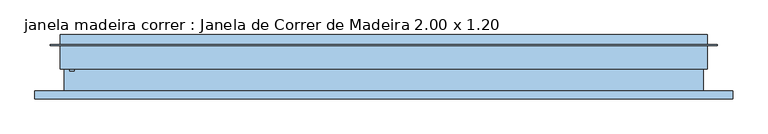
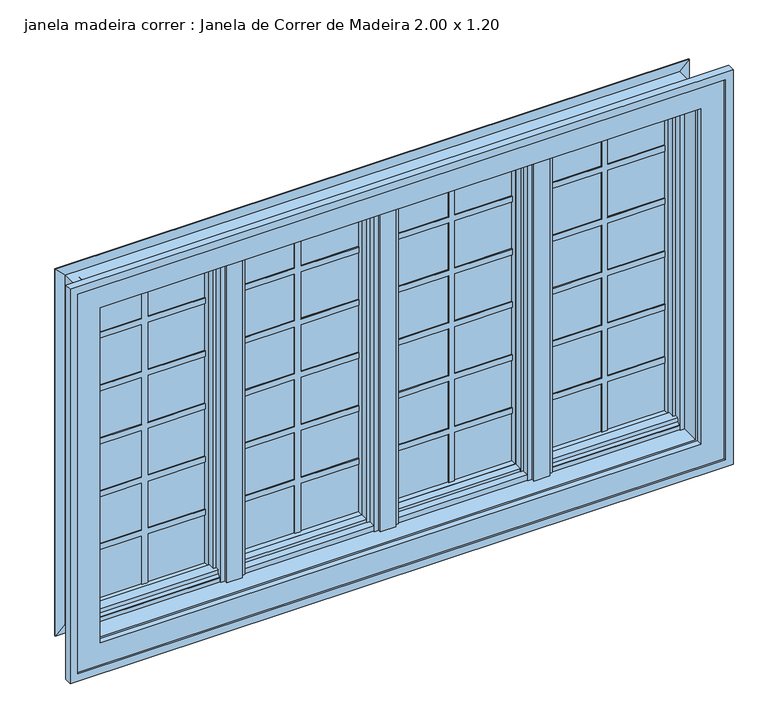
"""IFC4 building model written with IfcOpenShell, lengths in millimetres: window geometry, janela madeira correr : Janela de Correr de Madeira 2.00 x 1.20."""

from ifc_helpers import new_model, si_unit, frame, origin, place, context, project, spatial, polyline, outline, extrude, faceted_brep, source, transform, mapped, element, save


def janela_madeira_correr_janela_de_correr_de_madeira_2_00_x_1_d447c460(model_context):
    return source(origin(), model_context, "Body", "SolidModel", [
        extrude(outline(polyline([(1881.6300584, 206.5264803), (1881.6300584, 13.2337398), (1862.5800584, 13.2337398), (1862.5800584, 206.5264803), (1699.6775292, 206.5264803), (1699.6775292, 13.2337398), (1680.6275292, 13.2337398), (1680.6275292, 206.5264803), (1517.725, 206.5264803), (1517.725, 13.2337398), (1498.675, 13.2337398), (1498.675, 206.5264803), (1335.7724708, 206.5264803), (1335.7724708, 13.2337398), (1316.7224708, 13.2337398), (1316.7224708, 206.5264803), (1153.8199416, 206.5264803), (1153.8199416, 13.2337398), (1134.7699416, 13.2337398), (1134.7699416, 206.5264803), (962.3424123, 206.5264803), (962.3424123, 225.5764803), (1134.7699416, 225.5764803), (1134.7699416, 418.8692207), (1153.8199416, 418.8692207), (1153.8199416, 225.5764803), (1316.7224708, 225.5764803), (1316.7224708, 418.8692207), (1335.7724708, 418.8692207), (1335.7724708, 225.5764803), (1498.675, 225.5764803), (1498.675, 418.8692207), (1517.725, 418.8692207), (1517.725, 225.5764803), (1680.6275292, 225.5764803), (1680.6275292, 418.8692207), (1699.6775292, 418.8692207), (1699.6775292, 225.5764803), (1862.5800584, 225.5764803), (1862.5800584, 418.8692207), (1881.6300584, 418.8692207), (1881.6300584, 225.5764803), (2054.0575877, 225.5764803), (2054.0575877, 206.5264803), (1881.6300584, 206.5264803)])), frame((0.0, 46.9582456, 0.0), z_axis=(0.0, 1.0, 0.0), x_axis=(0.0, 0.0, 1.0)), (0.0, 0.0, 1.0), 3.1432544),
        extrude(outline(polyline([(1881.6300584, -293.4735197), (1881.6300584, -486.7662602), (1862.5800584, -486.7662602), (1862.5800584, -293.4735197), (1699.6775292, -293.4735197), (1699.6775292, -486.7662602), (1680.6275292, -486.7662602), (1680.6275292, -293.4735197), (1517.725, -293.4735197), (1517.725, -486.7662602), (1498.675, -486.7662602), (1498.675, -293.4735197), (1335.7724708, -293.4735197), (1335.7724708, -486.7662602), (1316.7224708, -486.7662602), (1316.7224708, -293.4735197), (1153.8199416, -293.4735197), (1153.8199416, -486.7662602), (1134.7699416, -486.7662602), (1134.7699416, -293.4735197), (962.3424123, -293.4735197), (962.3424123, -274.4235197), (1134.7699416, -274.4235197), (1134.7699416, -81.1307793), (1153.8199416, -81.1307793), (1153.8199416, -274.4235197), (1316.7224708, -274.4235197), (1316.7224708, -81.1307793), (1335.7724708, -81.1307793), (1335.7724708, -274.4235197), (1498.675, -274.4235197), (1498.675, -81.1307793), (1517.725, -81.1307793), (1517.725, -274.4235197), (1680.6275292, -274.4235197), (1680.6275292, -81.1307793), (1699.6775292, -81.1307793), (1699.6775292, -274.4235197), (1862.5800584, -274.4235197), (1862.5800584, -81.1307793), (1881.6300584, -81.1307793), (1881.6300584, -274.4235197), (2054.0575877, -274.4235197), (2054.0575877, -293.4735197), (1881.6300584, -293.4735197)])), frame((0.0, 46.9582456, 0.0), z_axis=(0.0, 1.0, 0.0), x_axis=(0.0, 0.0, 1.0)), (0.0, 0.0, 1.0), 3.1432544),
        extrude(outline(polyline([(1881.6300584, 206.5264803), (1881.6300584, 13.2337398), (1862.5800584, 13.2337398), (1862.5800584, 206.5264803), (1699.6775292, 206.5264803), (1699.6775292, 13.2337398), (1680.6275292, 13.2337398), (1680.6275292, 206.5264803), (1517.725, 206.5264803), (1517.725, 13.2337398), (1498.675, 13.2337398), (1498.675, 206.5264803), (1335.7724708, 206.5264803), (1335.7724708, 13.2337398), (1316.7224708, 13.2337398), (1316.7224708, 206.5264803), (1153.6503822, 206.5264803), (1153.6503822, 13.2337398), (1134.6003822, 13.2337398), (1134.6003822, 206.5264803), (962.3424123, 206.5264803), (962.3424123, 225.5764803), (1134.6003822, 225.5764803), (1134.6003822, 418.8692207), (1153.6503822, 418.8692207), (1153.6503822, 225.5764803), (1316.7224708, 225.5764803), (1316.7224708, 418.8692207), (1335.7724708, 418.8692207), (1335.7724708, 225.5764803), (1498.675, 225.5764803), (1498.675, 418.8692207), (1517.725, 418.8692207), (1517.725, 225.5764803), (1680.6275292, 225.5764803), (1680.6275292, 418.8692207), (1699.6775292, 418.8692207), (1699.6775292, 225.5764803), (1862.5800584, 225.5764803), (1862.5800584, 418.8692207), (1881.6300584, 418.8692207), (1881.6300584, 225.5764803), (2054.0575877, 225.5764803), (2054.0575877, 206.5264803), (1881.6300584, 206.5264803)])), frame((0.0, 50.1015, 0.0), z_axis=(0.0, 1.0, 0.0), x_axis=(0.0, 0.0, 1.0)), (0.0, 0.0, 1.0), 15.875),
        extrude(outline(polyline([(1881.6300584, -293.4735197), (1881.6300584, -486.7662602), (1862.5800584, -486.7662602), (1862.5800584, -293.4735197), (1699.6775292, -293.4735197), (1699.6775292, -486.7662602), (1680.6275292, -486.7662602), (1680.6275292, -293.4735197), (1517.725, -293.4735197), (1517.725, -486.7662602), (1498.675, -486.7662602), (1498.675, -293.4735197), (1335.7724708, -293.4735197), (1335.7724708, -486.7662602), (1316.7224708, -486.7662602), (1316.7224708, -293.4735197), (1153.8199416, -293.4735197), (1153.8199416, -486.7662602), (1134.7699416, -486.7662602), (1134.7699416, -293.4735197), (962.3424123, -293.4735197), (962.3424123, -274.4235197), (1134.7699416, -274.4235197), (1134.7699416, -81.1307793), (1153.8199416, -81.1307793), (1153.8199416, -274.4235197), (1316.7224708, -274.4235197), (1316.7224708, -81.1307793), (1335.7724708, -81.1307793), (1335.7724708, -274.4235197), (1498.675, -274.4235197), (1498.675, -81.1307793), (1517.725, -81.1307793), (1517.725, -274.4235197), (1680.6275292, -274.4235197), (1680.6275292, -81.1307793), (1699.6775292, -81.1307793), (1699.6775292, -274.4235197), (1862.5800584, -274.4235197), (1862.5800584, -81.1307793), (1881.6300584, -81.1307793), (1881.6300584, -274.4235197), (2054.0575877, -274.4235197), (2054.0575877, -293.4735197), (1881.6300584, -293.4735197)])), frame((0.0, 50.1015, 0.0), z_axis=(0.0, 1.0, 0.0), x_axis=(0.0, 0.0, 1.0)), (0.0, 0.0, 1.0), 15.875),
        extrude(outline(polyline([(-79.1922697, 50.1015), (-488.7047697, 50.1015), (-488.7047697, 65.9765), (-79.1922697, 65.9765), (-79.1922697, 50.1015)])), frame((0.0, 0.0, 962.3424123), z_axis=(0.0, 0.0, 1.0), x_axis=(1.0, 0.0, 0.0)), (0.0, 0.0, 1.0), 1091.7151753),
        faceted_brep([(1019.5438803, -105.0, 855.00605), (1019.5438803, -98.65, 855.00605), (-1087.4409197, -98.65, 855.00605), (-1087.4409197, -105.0, 855.00605), (1044.9438803, -79.6, 829.60605), (1044.9438803, -105.0, 829.60605), (-1112.8409197, -105.0, 829.60605), (-1112.8409197, -79.6, 829.60605), (943.3438803, -98.65, 931.20605), (943.3438803, -79.6, 931.20605), (-1011.2409197, -79.6, 931.20605), (-1011.2409197, -98.65, 931.20605), (-1087.4409197, -98.65, 2161.72415), (-1087.4409197, -105.0, 2161.72415), (-1112.8409197, -105.0, 2187.12415), (-1112.8409197, -79.6, 2187.12415), (-1011.2409197, -79.6, 2085.52415), (-1011.2409197, -98.65, 2085.52415), (1019.5438803, -98.65, 2161.72415), (1019.5438803, -105.0, 2161.72415), (1044.9438803, -105.0, 2187.12415), (1044.9438803, -79.6, 2187.12415), (943.3438803, -79.6, 2085.52415), (943.3438803, -98.65, 2085.52415)], [[[0, 1, 2, 3]], [[4, 5, 6, 7]], [[8, 9, 10, 11]], [[3, 2, 12, 13]], [[7, 6, 14, 15]], [[11, 10, 16, 17]], [[13, 12, 18, 19]], [[15, 14, 20, 21]], [[17, 16, 22, 23]], [[1, 18, 12, 2], [11, 17, 23, 8]], [[19, 18, 1, 0]], [[5, 20, 14, 6], [3, 13, 19, 0]], [[21, 20, 5, 4]], [[7, 15, 21, 4], [9, 22, 16, 10]], [[23, 22, 9, 8]]]),
        extrude(outline(polyline([(1153.8199416, 723.716552), (1316.7224708, 723.716552), (1316.7224708, 917.0878737), (1335.7724708, 917.0878737), (1335.7724708, 723.716552), (1498.675, 723.716552), (1498.675, 917.0878737), (1517.725, 917.0878737), (1517.725, 723.716552), (1680.6275292, 723.716552), (1680.6275292, 917.0878737), (1699.6775292, 917.0878737), (1699.6775292, 723.716552), (1862.5800584, 723.716552), (1862.5800584, 917.0878737), (1881.6300584, 917.0878737), (1881.6300584, 723.716552), (2054.0575877, 723.716552), (2054.0575877, 704.666552), (1881.6300584, 704.666552), (1881.6300584, 511.2952303), (1862.5800584, 511.2952303), (1862.5800584, 704.666552), (1699.6775292, 704.666552), (1699.6775292, 511.2952303), (1680.6275292, 511.2952303), (1680.6275292, 704.666552), (1517.725, 704.666552), (1517.725, 511.2952303), (1498.675, 511.2952303), (1498.675, 704.666552), (1335.7724708, 704.666552), (1335.7724708, 511.2952303), (1316.7224708, 511.2952303), (1316.7224708, 704.666552), (1153.8199416, 704.666552), (1153.8199416, 511.2952303), (1134.7699416, 511.2952303), (1134.7699416, 704.666552), (962.3424123, 704.666552), (962.3424123, 723.716552), (1134.7699416, 723.716552), (1134.7699416, 917.0878737), (1153.8199416, 917.0878737), (1153.8199416, 723.716552)])), frame((0.0, 46.7303732, 0.0), z_axis=(0.0, 1.0, 0.0), x_axis=(0.0, 0.0, 1.0)), (0.0, 0.0, 1.0), 3.3711268),
        extrude(outline(polyline([(1881.6300584, -791.6417168), (1881.6300584, -984.9344572), (1862.5800584, -984.9344572), (1862.5800584, -791.6417168), (1699.6775292, -791.6417168), (1699.6775292, -984.9344572), (1680.6275292, -984.9344572), (1680.6275292, -791.6417168), (1517.725, -791.6417168), (1517.725, -984.9344572), (1498.675, -984.9344572), (1498.675, -791.6417168), (1335.7724708, -791.6417168), (1335.7724708, -984.9344572), (1316.7224708, -984.9344572), (1316.7224708, -791.6417168), (1153.8199416, -791.6417168), (1153.8199416, -984.9344572), (1134.7699416, -984.9344572), (1134.7699416, -791.6417168), (962.3424123, -791.6417168), (962.3424123, -772.5917168), (1134.7699416, -772.5917168), (1134.7699416, -579.2989763), (1153.8199416, -579.2989763), (1153.8199416, -772.5917168), (1316.7224708, -772.5917168), (1316.7224708, -579.2989763), (1335.7724708, -579.2989763), (1335.7724708, -772.5917168), (1498.675, -772.5917168), (1498.675, -579.2989763), (1517.725, -579.2989763), (1517.725, -772.5917168), (1680.6275292, -772.5917168), (1680.6275292, -579.2989763), (1699.6775292, -579.2989763), (1699.6775292, -772.5917168), (1862.5800584, -772.5917168), (1862.5800584, -579.2989763), (1881.6300584, -579.2989763), (1881.6300584, -772.5917168), (2054.0575877, -772.5917168), (2054.0575877, -791.6417168), (1881.6300584, -791.6417168)])), frame((0.0, 46.9582456, 0.0), z_axis=(0.0, 1.0, 0.0), x_axis=(0.0, 0.0, 1.0)), (0.0, 0.0, 1.0), 3.1432544),
        extrude(outline(polyline([(35.1373, 2049.7546), (9.8065079, 2049.7546), (9.2928, 2058.8986), (-15.6627, 2058.8986), (-15.6627, 2079.17415), (-11.7892, 2079.17415), (-11.7892, 2072.0304), (35.1373, 2072.0304), (35.1373, 2049.7546)])), frame((-494.6547197, 0.0, 0.0), z_axis=(1.0, 0.0, 0.0), x_axis=(0.0, 1.0, 0.0)), (0.0, 0.0, 1.0), 921.4124),
        extrude(outline(polyline([(35.1373, 965.477), (35.1373, 944.3696), (-11.7892, 944.3696), (-11.7892, 937.55605), (-15.6627, 937.55605), (-15.6627, 955.952), (9.0471115, 955.952), (9.8065079, 965.477), (35.1373, 965.477)])), frame((-494.6547197, 0.0, 0.0), z_axis=(1.0, 0.0, 0.0), x_axis=(0.0, 1.0, 0.0)), (0.0, 0.0, 1.0), 921.4124),
        extrude(outline(polyline([(35.1373, 2049.7546), (9.8065079, 2049.7546), (9.2928, 2058.8986), (-15.6627, 2058.8986), (-15.6627, 2079.17415), (-11.7892, 2079.17415), (-11.7892, 2072.0304), (35.1373, 2072.0304), (35.1373, 2049.7546)])), frame((-990.9971197, 0.0, 0.0), z_axis=(1.0, 0.0, 0.0), x_axis=(0.0, 1.0, 0.0)), (0.0, 0.0, 1.0), 417.6462326),
        extrude(outline(polyline([(35.1373, 965.477), (35.1373, 944.3696), (-11.7892, 944.3696), (-11.7892, 937.55605), (-15.6627, 937.55605), (-15.6627, 951.5578), (-12.2972, 951.5578), (-5.0582, 959.4826), (-3.9768196, 973.0462), (27.9364, 973.0462), (35.1373, 965.477)])), frame((-990.9971197, 0.0, 0.0), z_axis=(1.0, 0.0, 0.0), x_axis=(0.0, 1.0, 0.0)), (0.0, 0.0, 1.0), 417.6462326),
        faceted_brep([(454.9389803, 85.9373, 2088.2955442), (454.9389803, 48.6374, 2088.2955442), (454.9389803, 48.6374, 2069.8909496), (454.9389803, 35.1373, 2067.5291599), (454.9389803, 35.1373, 2050.1057516), (454.9389803, 48.6374, 2047.8865571), (454.9389803, 48.6374, 968.5290777), (454.9389803, 35.1373, 966.3098832), (454.9389803, 35.1373, 948.8864749), (454.9389803, 48.6374, 946.5246852), (454.9389803, 48.6374, 928.1044558), (454.9389803, 85.9373, 928.1044558), (-23.7161471, 85.9373, 2088.2955442), (-23.7161471, 85.9373, 2059.2701124), (-23.7161471, 74.7560374, 2057.8452835), (-23.7161471, 74.4029109, 2047.2338554), (-23.7161471, 69.3765, 2044.5482224), (-23.7161471, 69.3765, 2060.523579), (-23.7161471, 53.5015, 2060.523579), (-23.7161471, 53.5015, 2047.086979), (-23.7161471, 35.1373, 2050.1057516), (-23.7161471, 35.1373, 2067.5291599), (-23.7161471, 48.6374, 2069.8909496), (-23.7161471, 48.6374, 2088.2955442), (-23.7161471, 53.5015, 969.3286558), (-23.7161471, 53.5015, 955.8920558), (-23.7161471, 69.3765, 955.8920558), (-23.7161471, 69.3765, 971.8674123), (-23.7161471, 74.4029109, 969.1817794), (-23.7161471, 74.7560374, 958.5703513), (-23.7161471, 85.9373, 957.1455224), (-23.7161471, 85.9373, 928.1044558), (-23.7161471, 48.6374, 928.1044558), (-23.7161471, 48.6374, 946.5246852), (-23.7161471, 35.1373, 948.8864749), (-23.7161471, 35.1373, 966.3098832), (-4.4157903, 48.6374, 2088.2955442), (-2.0540006, 35.1373, 2088.2955442), (15.3694077, 35.1373, 2088.2955442), (17.5886022, 48.6374, 2088.2955442), (414.5143584, 48.6374, 2088.2955442), (416.7335529, 35.1373, 2088.2955442), (434.1569612, 35.1373, 2088.2955442), (436.5187509, 48.6374, 2088.2955442), (436.5187509, 48.6374, 2069.8909496), (-22.8360197, 48.6374, 2069.8909496), (-4.4157903, 48.6374, 2069.8909496), (17.5886022, 48.6374, 2069.8909496), (414.5143584, 48.6374, 2069.8909496), (434.1569612, 35.1373, 2067.5291599), (-2.0540006, 35.1373, 2067.5291599), (15.3694077, 35.1373, 2067.5291599), (416.7335529, 35.1373, 2067.5291599), (-2.0540006, 35.1373, 928.1044558), (15.3694077, 35.1373, 928.1044558), (15.3694077, 35.1373, 948.8864749), (416.7335529, 35.1373, 948.8864749), (416.7335529, 35.1373, 928.1044558), (434.1569612, 35.1373, 928.1044558), (434.1569612, 35.1373, 948.8864749), (434.1569612, 35.1373, 966.3098832), (434.1569612, 35.1373, 2050.1057516), (-2.0540006, 35.1373, 2050.1057516), (-2.0540006, 35.1373, 966.3098832), (-2.0540006, 35.1373, 948.8864749), (416.7335529, 35.1373, 2050.1057516), (416.7335529, 35.1373, 966.3098832), (15.3694077, 35.1373, 966.3098832), (15.3694077, 35.1373, 2050.1057516), (436.5187509, 48.6374, 2047.8865571), (-22.8360197, 53.5015, 2047.086979), (-22.8360197, 48.6374, 2047.8865571), (-4.4157903, 48.6374, 2047.8865571), (18.3881803, 53.5015, 2047.086979), (413.7147803, 53.5015, 2047.086979), (-22.8360197, 53.5015, 2060.523579), (-22.8360197, 53.5015, 969.3286558), (-22.8360197, 53.5015, 955.8920558), (427.1513803, 53.5015, 2060.523579), (427.1513803, 53.5015, 955.8920558), (4.9515803, 53.5015, 955.8920558), (4.9515803, 53.5015, 2060.523579), (18.3881803, 53.5015, 969.3286558), (413.7147803, 53.5015, 969.3286558), (-22.8360197, 69.3765, 2060.523579), (4.9515803, 69.3765, 2060.523579), (427.1513803, 69.3765, 2060.523579), (-22.8360197, 69.3765, 2044.5482224), (-22.8360197, 69.3765, 955.8920558), (-22.8360197, 69.3765, 971.8674123), (4.9515803, 69.3765, 955.8920558), (427.1513803, 69.3765, 955.8920558), (411.1760237, 69.3765, 2044.5482224), (411.1760237, 69.3765, 971.8674123), (20.9269368, 69.3765, 971.8674123), (20.9269368, 69.3765, 2044.5482224), (-22.8360197, 74.4029109, 2047.2338554), (18.2413039, 74.4029109, 2047.2338554), (413.8616566, 74.4029109, 2047.2338554), (-22.8360197, 74.7560374, 2057.8452835), (7.6298758, 74.7560374, 2057.8452835), (424.4730847, 74.7560374, 2057.8452835), (-22.8360197, 85.9373, 2059.2701124), (6.2050469, 85.9373, 2059.2701124), (425.8979136, 85.9373, 2059.2701124), (-22.8360197, 85.9373, 957.1455224), (6.2050469, 85.9373, 957.1455224), (425.8979136, 85.9373, 957.1455224), (436.5187509, 48.6374, 968.5290777), (-4.4157903, 48.6374, 968.5290777), (-22.8360197, 48.6374, 968.5290777), (436.5187509, 48.6374, 946.5246852), (-22.8360197, 48.6374, 946.5246852), (-4.4157903, 48.6374, 946.5246852), (17.5886022, 48.6374, 946.5246852), (414.5143584, 48.6374, 946.5246852), (436.5187509, 48.6374, 928.1044558), (-4.4157903, 48.6374, 928.1044558), (17.5886022, 48.6374, 928.1044558), (414.5143584, 48.6374, 928.1044558), (-22.8360197, 74.7560374, 958.5703513), (7.6298758, 74.7560374, 958.5703513), (424.4730847, 74.7560374, 958.5703513), (-22.8360197, 74.4029109, 969.1817794), (18.2413039, 74.4029109, 969.1817794), (413.8616566, 74.4029109, 969.1817794)], [[[0, 1, 2, 3, 4, 5, 6, 7, 8, 9, 10, 11]], [[12, 13, 14, 15, 16, 17, 18, 19, 20, 21, 22, 23]], [[24, 25, 26, 27, 28, 29, 30, 31, 32, 33, 34, 35]], [[1, 0, 12, 23, 36, 37, 38, 39, 40, 41, 42, 43]], [[2, 1, 43, 44]], [[36, 23, 22, 45, 46]], [[40, 39, 47, 48]], [[3, 2, 44, 49]], [[22, 21, 50, 46, 45]], [[48, 47, 51, 52]], [[53, 54, 55, 56, 57, 58, 59, 8, 7, 60, 61, 4, 3, 49, 42, 41, 52, 51, 38, 37, 50, 21, 20, 62, 63, 35, 34, 64], [65, 66, 67, 68]], [[5, 4, 61, 69]], [[20, 19, 70, 71, 72, 62]], [[65, 68, 73, 74]], [[19, 18, 75, 70]], [[25, 24, 76, 77]], [[78, 79, 80, 81], [74, 73, 82, 83]], [[18, 17, 84, 75]], [[78, 81, 85, 86]], [[17, 16, 87, 84]], [[27, 26, 88, 89]], [[86, 85, 90, 91], [92, 93, 94, 95]], [[16, 15, 96, 87]], [[92, 95, 97, 98]], [[15, 14, 99, 96]], [[98, 97, 100, 101]], [[14, 13, 102, 99]], [[101, 100, 103, 104]], [[12, 0, 11, 31, 30, 105, 102, 13], [103, 106, 107, 104]], [[7, 6, 108, 60]], [[24, 35, 63, 109, 110, 76]], [[83, 82, 67, 66]], [[9, 8, 59, 111]], [[34, 33, 112, 113, 64]], [[56, 55, 114, 115]], [[10, 9, 111, 116]], [[33, 32, 117, 113, 112]], [[115, 114, 118, 119]], [[31, 11, 10, 116, 58, 57, 119, 118, 54, 53, 117, 32]], [[30, 29, 120, 105]], [[107, 106, 121, 122]], [[29, 28, 123, 120]], [[122, 121, 124, 125]], [[28, 27, 89, 123]], [[125, 124, 94, 93]], [[26, 25, 77, 88]], [[91, 90, 80, 79]], [[101, 122, 125, 98]], [[104, 107, 122, 101]], [[6, 5, 69, 108]], [[43, 42, 49, 44]], [[61, 60, 108, 69]], [[58, 116, 111, 59]], [[41, 40, 48, 52]], [[57, 56, 115, 119]], [[74, 83, 66, 65]], [[79, 78, 86, 91]], [[98, 125, 93, 92]], [[124, 97, 95, 94]], [[81, 80, 90, 85]], [[39, 38, 51, 47]], [[55, 54, 118, 114]], [[82, 73, 68, 67]], [[37, 36, 46, 50]], [[63, 62, 72, 109]], [[117, 53, 64, 113]], [[109, 72, 71, 110]], [[102, 105, 120, 123, 89, 88, 77, 76, 110, 71, 70, 75, 84, 87, 96, 99]], [[106, 103, 100, 121]], [[121, 100, 97, 124]]]),
        faceted_brep([(-86.1383434, 74.4029109, 2088.2955442), (-88.8239763, 69.3765, 2088.2955442), (-72.8486197, 69.3765, 2088.2955442), (-72.8486197, 53.5015, 2088.2955442), (-86.2852197, 53.5015, 2088.2955442), (-83.2664471, 35.1373, 2088.2955442), (-65.8430388, 35.1373, 2088.2955442), (-63.4812491, 48.6374, 2088.2955442), (-45.0610197, 48.6374, 2088.2955442), (-45.0610197, 85.9373, 2088.2955442), (-74.1020864, 85.9373, 2088.2955442), (-75.5269153, 74.7560374, 2088.2955442), (-86.1383434, 74.4029109, 928.1044558), (-75.5269153, 74.7560374, 928.1044558), (-74.1020864, 85.9373, 928.1044558), (-45.0610197, 85.9373, 928.1044558), (-45.0610197, 48.6374, 928.1044558), (-63.4812491, 48.6374, 928.1044558), (-65.8430388, 35.1373, 928.1044558), (-83.2664471, 35.1373, 928.1044558), (-86.2852197, 53.5015, 928.1044558), (-72.8486197, 53.5015, 928.1044558), (-72.8486197, 69.3765, 928.1044558), (-88.8239763, 69.3765, 928.1044558)], [[[0, 1, 2, 3, 4, 5, 6, 7, 8, 9, 10, 11]], [[12, 13, 14, 15, 16, 17, 18, 19, 20, 21, 22, 23]], [[13, 12, 0, 11]], [[14, 13, 11, 10]], [[15, 14, 10, 9]], [[16, 15, 9, 8]], [[17, 16, 8, 7]], [[18, 17, 7, 6]], [[19, 18, 6, 5]], [[20, 19, 5, 4]], [[21, 20, 4, 3]], [[22, 21, 3, 2]], [[23, 22, 2, 1]], [[12, 23, 1, 0]]]),
        faceted_brep([(-481.7586961, 74.4029109, 2088.2955442), (-492.3701242, 74.7560374, 2088.2955442), (-493.7949531, 85.9373, 2088.2955442), (-522.8360197, 85.9373, 2088.2955442), (-522.8360197, 48.6374, 2088.2955442), (-504.4157903, 48.6374, 2088.2955442), (-502.0540006, 35.1373, 2088.2955442), (-484.6305923, 35.1373, 2088.2955442), (-481.6118197, 53.5015, 2088.2955442), (-495.0484197, 53.5015, 2088.2955442), (-495.0484197, 69.3765, 2088.2955442), (-479.0730632, 69.3765, 2088.2955442), (-481.7586961, 74.4029109, 928.1044558), (-479.0730632, 69.3765, 928.1044558), (-495.0484197, 69.3765, 928.1044558), (-495.0484197, 53.5015, 928.1044558), (-481.6118197, 53.5015, 928.1044558), (-484.6305923, 35.1373, 928.1044558), (-502.0540006, 35.1373, 928.1044558), (-504.4157903, 48.6374, 928.1044558), (-522.8360197, 48.6374, 928.1044558), (-522.8360197, 85.9373, 928.1044558), (-493.7949531, 85.9373, 928.1044558), (-492.3701242, 74.7560374, 928.1044558)], [[[0, 1, 2, 3, 4, 5, 6, 7, 8, 9, 10, 11]], [[12, 13, 14, 15, 16, 17, 18, 19, 20, 21, 22, 23]], [[13, 12, 0, 11]], [[14, 13, 11, 10]], [[15, 14, 10, 9]], [[16, 15, 9, 8]], [[17, 16, 8, 7]], [[18, 17, 7, 6]], [[19, 18, 6, 5]], [[20, 19, 5, 4]], [[21, 20, 4, 3]], [[22, 21, 3, 2]], [[23, 22, 2, 1]], [[12, 23, 1, 0]]]),
        extrude(outline(polyline([(35.1373, 2049.7546), (9.8065079, 2049.7546), (9.2928, 2058.8986), (-15.6627, 2058.8986), (-15.6627, 2079.17415), (-11.7892, 2079.17415), (-11.7892, 2072.0304), (35.1373, 2072.0304), (35.1373, 2049.7546)])), frame((502.0932267, 0.0, 0.0), z_axis=(1.0, 0.0, 0.0), x_axis=(0.0, 1.0, 0.0)), (0.0, 0.0, 1.0), 424.1385817),
        extrude(outline(polyline([(35.1373, 965.477), (35.1373, 944.3696), (-11.7892, 944.3696), (-11.7892, 937.55605), (-15.6627, 937.55605), (-15.6627, 951.5578), (-12.2972, 951.5578), (-5.0582, 959.4826), (-3.9768196, 973.0462), (27.9364, 973.0462), (35.1373, 965.477)])), frame((502.0932267, 0.0, 0.0), z_axis=(1.0, 0.0, 0.0), x_axis=(0.0, 1.0, 0.0)), (0.0, 0.0, 1.0), 424.1385817),
        extrude(outline(polyline([(-59.3485197, 32.1945), (-59.3485197, -19.05), (-73.2423197, -19.05), (-73.2423197, 6.35), (-82.3863197, 6.8637079), (-82.3863197, 32.1945), (-59.3485197, 32.1945)])), frame((0.0, 0.0, 937.55605), z_axis=(0.0, 0.0, 1.0), x_axis=(1.0, 0.0, 0.0)), (0.0, 0.0, 1.0), 1141.6181),
        extrude(outline(polyline([(-8.5485197, 32.1945), (14.4892803, 32.1945), (14.4892803, 6.8637079), (5.3452803, 6.35), (5.3452803, -19.05), (-8.5485197, -19.05), (-8.5485197, 32.1945)])), frame((0.0, 0.0, 937.55605), z_axis=(0.0, 0.0, 1.0), x_axis=(1.0, 0.0, 0.0)), (0.0, 0.0, 1.0), 1141.6181),
        extrude(outline(polyline([(420.8077303, 50.1015), (11.2952303, 50.1015), (11.2952303, 65.9765), (420.8077303, 65.9765), (420.8077303, 50.1015)])), frame((0.0, 0.0, 962.3424123), z_axis=(0.0, 0.0, 1.0), x_axis=(1.0, 0.0, 0.0)), (0.0, 0.0, 1.0), 1091.7151753),
        extrude(outline(polyline([(1153.8199416, 723.716552), (1316.7224708, 723.716552), (1316.7224708, 917.0878737), (1335.7724708, 917.0878737), (1335.7724708, 723.716552), (1498.675, 723.716552), (1498.675, 917.0878737), (1517.725, 917.0878737), (1517.725, 723.716552), (1680.6275292, 723.716552), (1680.6275292, 917.0878737), (1699.6775292, 917.0878737), (1699.6775292, 723.716552), (1862.5800584, 723.716552), (1862.5800584, 917.0878737), (1881.6300584, 917.0878737), (1881.6300584, 723.716552), (2054.0575877, 723.716552), (2054.0575877, 704.666552), (1881.6300584, 704.666552), (1881.6300584, 511.2952303), (1862.5800584, 511.2952303), (1862.5800584, 704.666552), (1699.6775292, 704.666552), (1699.6775292, 511.2952303), (1680.6275292, 511.2952303), (1680.6275292, 704.666552), (1517.725, 704.666552), (1517.725, 511.2952303), (1498.675, 511.2952303), (1498.675, 704.666552), (1335.7724708, 704.666552), (1335.7724708, 511.2952303), (1316.7224708, 511.2952303), (1316.7224708, 704.666552), (1153.8199416, 704.666552), (1153.8199416, 511.2952303), (1134.7699416, 511.2952303), (1134.7699416, 704.666552), (962.3424123, 704.666552), (962.3424123, 723.716552), (1134.7699416, 723.716552), (1134.7699416, 917.0878737), (1153.8199416, 917.0878737), (1153.8199416, 723.716552)])), frame((0.0, 50.1015, 0.0), z_axis=(0.0, 1.0, 0.0), x_axis=(0.0, 0.0, 1.0)), (0.0, 0.0, 1.0), 15.875),
        extrude(outline(polyline([(917.0878737, 50.1015), (511.2952303, 50.1015), (511.2952303, 65.9765), (917.0878737, 65.9765), (917.0878737, 50.1015)])), frame((0.0, 0.0, 962.3424123), z_axis=(0.0, 0.0, 1.0), x_axis=(1.0, 0.0, 0.0)), (0.0, 0.0, 1.0), 1091.8825877),
        extrude(outline(polyline([(440.6514803, -3.9768196), (440.6514803, 48.6374), (455.8191077, 48.6374), (459.7768673, 93.8748), (472.3260932, 93.8748), (476.2838529, 48.6374), (491.4514803, 48.6374), (491.4514803, -3.9768196), (440.6514803, -3.9768196)])), frame((0.0, 0.0, 925.6747737), z_axis=(0.0, 0.0, 1.0), x_axis=(1.0, 0.0, 0.0)), (0.0, 0.0, 1.0), 1165.0504526),
        extrude(outline(polyline([(-559.3485197, -3.9768196), (-559.3485197, 48.6374), (-544.1808923, 48.6374), (-540.2231327, 93.8748), (-527.6739068, 93.8748), (-523.7161471, 48.6374), (-508.5485197, 48.6374), (-508.5485197, -3.9768196), (-559.3485197, -3.9768196)])), frame((0.0, 0.0, 925.6747737), z_axis=(0.0, 0.0, 1.0), x_axis=(1.0, 0.0, 0.0)), (0.0, 0.0, 1.0), 1165.0504526),
        extrude(outline(polyline([(-59.3485197, -3.9768196), (-59.3485197, 48.6374), (-44.1808923, 48.6374), (-40.2231327, 93.8748), (-27.6739068, 93.8748), (-23.7161471, 48.6374), (-8.5485197, 48.6374), (-8.5485197, -3.9768196), (-59.3485197, -3.9768196)])), frame((0.0, 0.0, 925.6747737), z_axis=(0.0, 0.0, 1.0), x_axis=(1.0, 0.0, 0.0)), (0.0, 0.0, 1.0), 1165.0504526),
        faceted_brep([(951.3258303, 85.9373, 928.1044558), (951.3258303, 48.6374, 928.1044558), (932.9056009, 48.6374, 928.1044558), (930.5438112, 35.1373, 928.1044558), (913.1204029, 35.1373, 928.1044558), (910.9012084, 48.6374, 928.1044558), (517.5886022, 48.6374, 928.1044558), (515.3694077, 35.1373, 928.1044558), (497.9459994, 35.1373, 928.1044558), (495.5842097, 48.6374, 928.1044558), (477.1639803, 48.6374, 928.1044558), (477.1639803, 85.9373, 928.1044558), (913.1204029, 35.1373, 2079.6498291), (930.5438112, 35.1373, 2079.6498291), (932.9056009, 48.6374, 2079.6498291), (910.9012084, 48.6374, 2079.6498291), (495.5842097, 48.6374, 2079.6498291), (497.9459994, 35.1373, 2079.6498291), (515.3694077, 35.1373, 2079.6498291), (517.5886022, 48.6374, 2079.6498291), (910.2485066, 74.4029109, 969.1817794), (910.2485066, 74.4029109, 2047.2338554), (920.8599347, 74.7560374, 2057.8452835), (920.8599347, 74.7560374, 958.5703513), (922.2847636, 85.9373, 2059.2701124), (922.2847636, 85.9373, 957.1455224), (477.1639803, 85.9373, 2088.2955442), (951.3258303, 85.9373, 2088.2955442), (506.2050469, 85.9373, 2059.2701124), (506.2050469, 85.9373, 957.1455224), (951.3258303, 48.6374, 2088.2955442), (951.3258303, 48.6374, 2069.8909496), (951.3258303, 35.1373, 2067.5291599), (951.3258303, 35.1373, 2050.1057516), (951.3258303, 48.6374, 2047.8865571), (951.3258303, 48.6374, 968.5290777), (951.3258303, 35.1373, 966.3098832), (951.3258303, 35.1373, 948.8864749), (951.3258303, 48.6374, 946.5246852), (932.9056009, 48.6374, 946.5246852), (495.5842097, 48.6374, 946.5246852), (477.1639803, 48.6374, 946.5246852), (477.1639803, 48.6374, 2088.2955442), (477.1639803, 48.6374, 2069.8909496), (495.5842097, 48.6374, 2069.8909496), (517.5886022, 48.6374, 2069.8909496), (910.9012084, 48.6374, 2069.8909496), (932.9056009, 48.6374, 2069.8909496), (932.9056009, 48.6374, 2047.8865571), (932.9056009, 48.6374, 968.5290777), (495.5842097, 48.6374, 968.5290777), (495.5842097, 48.6374, 2047.8865571), (477.1639803, 48.6374, 2047.8865571), (477.1639803, 48.6374, 968.5290777), (930.5438112, 35.1373, 948.8864749), (930.5438112, 35.1373, 2067.5291599), (930.5438112, 35.1373, 2050.1057516), (930.5438112, 35.1373, 966.3098832), (477.1639803, 35.1373, 966.3098832), (477.1639803, 35.1373, 948.8864749), (497.9459994, 35.1373, 948.8864749), (515.3694077, 35.1373, 948.8864749), (913.1204029, 35.1373, 948.8864749), (913.1204029, 35.1373, 2067.5291599), (515.3694077, 35.1373, 2067.5291599), (497.9459994, 35.1373, 2067.5291599), (477.1639803, 35.1373, 2067.5291599), (477.1639803, 35.1373, 2050.1057516), (497.9459994, 35.1373, 2050.1057516), (497.9459994, 35.1373, 966.3098832), (913.1204029, 35.1373, 966.3098832), (515.3694077, 35.1373, 966.3098832), (515.3694077, 35.1373, 2050.1057516), (913.1204029, 35.1373, 2050.1057516), (910.9012084, 48.6374, 946.5246852), (910.1016303, 53.5015, 2047.086979), (910.1016303, 53.5015, 969.3286558), (923.5382303, 53.5015, 955.8920558), (504.9515803, 53.5015, 955.8920558), (504.9515803, 53.5015, 2060.523579), (923.5382303, 53.5015, 2060.523579), (518.3881803, 53.5015, 2047.086979), (518.3881803, 53.5015, 969.3286558), (923.5382303, 69.3765, 2060.523579), (923.5382303, 69.3765, 955.8920558), (504.9515803, 69.3765, 2060.523579), (504.9515803, 69.3765, 955.8920558), (907.5628737, 69.3765, 971.8674123), (520.9269368, 69.3765, 971.8674123), (520.9269368, 69.3765, 2044.5482224), (907.5628737, 69.3765, 2044.5482224), (518.2413039, 74.4029109, 969.1817794), (518.2413039, 74.4029109, 2047.2338554), (517.5886022, 48.6374, 946.5246852), (507.6298758, 74.7560374, 2057.8452835), (507.6298758, 74.7560374, 958.5703513)], [[[0, 1, 2, 3, 4, 5, 6, 7, 8, 9, 10, 11]], [[12, 13, 14, 15]], [[16, 17, 18, 19]], [[20, 21, 22, 23]], [[23, 22, 24, 25]], [[0, 11, 26, 27], [24, 28, 29, 25]], [[1, 0, 27, 30, 31, 32, 33, 34, 35, 36, 37, 38]], [[2, 1, 38, 39]], [[10, 9, 40, 41]], [[31, 30, 42, 43, 44, 16, 19, 45, 46, 15, 14, 47]], [[35, 34, 48, 49]], [[50, 51, 52, 53]], [[3, 2, 39, 54]], [[14, 13, 55, 47]], [[49, 48, 56, 57]], [[58, 59, 60, 8, 7, 61, 62, 4, 3, 54, 37, 36, 57, 56, 33, 32, 55, 13, 12, 63, 64, 18, 17, 65, 66, 67, 68, 69], [70, 71, 72, 73]], [[5, 4, 62, 74]], [[12, 15, 46, 63]], [[70, 73, 75, 76]], [[77, 78, 79, 80], [76, 75, 81, 82]], [[77, 80, 83, 84]], [[84, 83, 85, 86], [87, 88, 89, 90]], [[21, 20, 87, 90]], [[91, 92, 89, 88]], [[86, 85, 79, 78]], [[7, 6, 93, 61]], [[19, 18, 64, 45]], [[82, 81, 72, 71]], [[9, 8, 60, 40]], [[17, 16, 44, 65]], [[69, 68, 51, 50]], [[26, 11, 10, 41, 59, 58, 53, 52, 67, 66, 43, 42]], [[29, 28, 94, 95]], [[92, 91, 95, 94]], [[30, 27, 26, 42]], [[32, 31, 47, 55]], [[64, 63, 46, 45]], [[43, 66, 65, 44]], [[34, 33, 56, 48]], [[68, 67, 52, 51]], [[81, 75, 73, 72]], [[85, 83, 80, 79]], [[92, 21, 90, 89]], [[21, 92, 94, 22]], [[28, 24, 22, 94]], [[36, 35, 49, 57]], [[58, 69, 50, 53]], [[76, 82, 71, 70]], [[38, 37, 54, 39]], [[62, 61, 93, 74]], [[59, 41, 40, 60]], [[6, 5, 74, 93]], [[25, 29, 95, 23]], [[91, 20, 23, 95]], [[20, 91, 88, 87]], [[84, 86, 78, 77]]]),
        extrude(outline(polyline([(-559.3485197, -28.8072), (-559.3485197, -3.9768196), (-508.5485197, -3.9768196), (-508.5485197, -28.8072), (-559.3485197, -28.8072)])), frame((0.0, 0.0, 937.55605), z_axis=(0.0, 0.0, 1.0), x_axis=(1.0, 0.0, 0.0)), (0.0, 0.0, 1.0), 1141.6181),
        extrude(outline(polyline([(491.4514803, -28.8072), (440.6514803, -28.8072), (440.6514803, -3.9768196), (491.4514803, -3.9768196), (491.4514803, -28.8072)])), frame((0.0, 0.0, 937.55605), z_axis=(0.0, 0.0, 1.0), x_axis=(1.0, 0.0, 0.0)), (0.0, 0.0, 1.0), 1141.6181),
        extrude(outline(polyline([(-8.5485197, -28.8072), (-59.3485197, -28.8072), (-59.3485197, -3.9768196), (-8.5485197, -3.9768196), (-8.5485197, -28.8072)])), frame((0.0, 0.0, 937.55605), z_axis=(0.0, 0.0, 1.0), x_axis=(1.0, 0.0, 0.0)), (0.0, 0.0, 1.0), 1141.6181),
        extrude(outline(polyline([(-579.2989763, 50.1015), (-984.9344572, 50.1015), (-984.9344572, 65.9765), (-579.2989763, 65.9765), (-579.2989763, 50.1015)])), frame((0.0, 0.0, 962.3424123), z_axis=(0.0, 0.0, 1.0), x_axis=(1.0, 0.0, 0.0)), (0.0, 0.0, 1.0), 1091.8825877),
        extrude(outline(polyline([(1881.6300584, -791.6417168), (1881.6300584, -984.9344572), (1862.5800584, -984.9344572), (1862.5800584, -791.6417168), (1699.6775292, -791.6417168), (1699.6775292, -984.9344572), (1680.6275292, -984.9344572), (1680.6275292, -791.6417168), (1517.725, -791.6417168), (1517.725, -984.9344572), (1498.675, -984.9344572), (1498.675, -791.6417168), (1335.7724708, -791.6417168), (1335.7724708, -984.9344572), (1316.7224708, -984.9344572), (1316.7224708, -791.6417168), (1153.8199416, -791.6417168), (1153.8199416, -984.9344572), (1134.7699416, -984.9344572), (1134.7699416, -791.6417168), (962.3424123, -791.6417168), (962.3424123, -772.5917168), (1134.7699416, -772.5917168), (1134.7699416, -579.2989763), (1153.8199416, -579.2989763), (1153.8199416, -772.5917168), (1316.7224708, -772.5917168), (1316.7224708, -579.2989763), (1335.7724708, -579.2989763), (1335.7724708, -772.5917168), (1498.675, -772.5917168), (1498.675, -579.2989763), (1517.725, -579.2989763), (1517.725, -772.5917168), (1680.6275292, -772.5917168), (1680.6275292, -579.2989763), (1699.6775292, -579.2989763), (1699.6775292, -772.5917168), (1862.5800584, -772.5917168), (1862.5800584, -579.2989763), (1881.6300584, -579.2989763), (1881.6300584, -772.5917168), (2054.0575877, -772.5917168), (2054.0575877, -791.6417168), (1881.6300584, -791.6417168)])), frame((0.0, 50.1015, 0.0), z_axis=(0.0, 1.0, 0.0), x_axis=(0.0, 0.0, 1.0)), (0.0, 0.0, 1.0), 15.875),
        faceted_brep([(966.0514803, -11.7892, 908.2), (966.0514803, 93.8748, 908.2), (966.0514803, 93.8748, 2108.2), (966.0514803, -11.7892, 2108.2), (-1033.9485197, -11.7892, 2108.2), (-1033.9485197, 93.8748, 2108.2), (-1033.9485197, 93.8748, 908.2), (-1033.9485197, -11.7892, 908.2), (936.9938803, -11.7892, 2072.0304), (936.9938803, -11.7892, 944.3696), (-1004.8909197, -11.7892, 944.3696), (-1004.8909197, -11.7892, 2072.0304), (-1004.8909197, 48.6374, 2072.0304), (936.9938803, 48.6374, 2072.0304), (953.7070803, 48.6374, 2090.7252263), (953.7070803, 48.6374, 925.6747737), (-1021.6041197, 48.6374, 925.6747737), (-1021.6041197, 48.6374, 2090.7252263), (-1004.8909197, 48.6374, 944.3696), (936.9938803, 48.6374, 944.3696), (-1021.6041197, 93.8748, 2090.7252263), (953.7070803, 93.8748, 2090.7252263), (-1021.6041197, 93.8748, 925.6747737), (953.7070803, 93.8748, 925.6747737)], [[[0, 1, 2, 3]], [[4, 5, 6, 7]], [[0, 3, 4, 7], [8, 9, 10, 11]], [[8, 11, 12, 13]], [[14, 15, 16, 17], [13, 12, 18, 19]], [[14, 17, 20, 21]], [[2, 1, 6, 5], [20, 22, 23, 21]], [[4, 3, 2, 5]], [[23, 22, 16, 15]], [[19, 18, 10, 9]], [[6, 1, 0, 7]], [[13, 19, 9, 8]], [[21, 23, 15, 14]], [[22, 20, 17, 16]], [[18, 12, 11, 10]]]),
        extrude(outline(polyline([(920.10625, 954.4436803), (2096.62395, 954.4436803), (2096.62395, -1022.3407197), (920.10625, -1022.3407197), (920.10625, 954.4436803)]), holes=[polyline([(2079.17415, 936.9938803), (937.55605, 936.9938803), (937.55605, -1004.8909197), (2079.17415, -1004.8909197), (2079.17415, 936.9938803)])]), frame((0.0, -79.6, 0.0), z_axis=(0.0, 1.0, 0.0), x_axis=(0.0, 0.0, 1.0)), (0.0, 0.0, 1.0), 67.8108),
        faceted_brep([(-551.4110197, 48.6374, 2069.8753148), (-551.4110197, 35.1373, 2067.5135251), (-551.4110197, 35.1373, 2050.0901168), (-551.4110197, 48.6374, 2047.3667015), (-551.4110197, 35.1373, 965.589539), (-551.4110197, 35.1373, 948.8864749), (-551.4110197, 48.6374, 946.5246852), (-551.4110197, 48.6374, 967.8087335), (-1019.2228697, 85.9373, 928.1044558), (-1019.2228697, 48.6374, 928.1044558), (-1019.2228697, 48.6374, 946.5246852), (-1019.2228697, 35.1373, 948.8864749), (-1019.2228697, 35.1373, 965.589539), (-1019.2228697, 48.6374, 967.8087335), (-1019.2228697, 48.6374, 2047.3667015), (-1019.2228697, 35.1373, 2050.0901168), (-1019.2228697, 35.1373, 2067.5135251), (-1019.2228697, 48.6374, 2069.8753148), (-1019.2228697, 48.6374, 2088.2955442), (-1019.2228697, 85.9373, 2088.2955442), (-1000.8026403, 48.6374, 2088.2955442), (-998.4408506, 35.1373, 2088.2955442), (-981.0174423, 35.1373, 2088.2955442), (-978.7982478, 48.6374, 2088.2955442), (-585.4856416, 48.6374, 2088.2955442), (-583.2664471, 35.1373, 2088.2955442), (-565.8430388, 35.1373, 2088.2955442), (-563.4812491, 48.6374, 2088.2955442), (-545.0610197, 48.6374, 2088.2955442), (-545.0610197, 85.9373, 2088.2955442), (-1000.8026403, 48.6374, 928.1044558), (-1000.8026403, 48.6374, 946.5246852), (-1000.8026403, 48.6374, 2069.8753148), (-978.7982478, 48.6374, 2069.8753148), (-585.4856416, 48.6374, 2069.8753148), (-563.4812491, 48.6374, 2069.8753148), (-563.4812491, 48.6374, 2047.3667015), (-563.4812491, 48.6374, 967.8087335), (-563.4812491, 48.6374, 946.5246852), (-563.4812491, 48.6374, 928.1044558), (-545.0610197, 48.6374, 928.1044558), (-585.4856416, 48.6374, 946.5246852), (-978.7982478, 48.6374, 946.5246852), (-978.7982478, 48.6374, 928.1044558), (-585.4856416, 48.6374, 928.1044558), (-565.8430388, 35.1373, 2067.5135251), (-998.4408506, 35.1373, 2067.5135251), (-981.0174423, 35.1373, 2067.5135251), (-583.2664471, 35.1373, 2067.5135251), (-583.2664471, 35.1373, 928.1044558), (-565.8430388, 35.1373, 928.1044558), (-565.8430388, 35.1373, 948.8864749), (-565.8430388, 35.1373, 965.589539), (-565.8430388, 35.1373, 2050.0901168), (-998.4408506, 35.1373, 2050.0901168), (-998.4408506, 35.1373, 965.589539), (-998.4408506, 35.1373, 948.8864749), (-998.4408506, 35.1373, 928.1044558), (-981.0174423, 35.1373, 928.1044558), (-981.0174423, 35.1373, 948.8864749), (-583.2664471, 35.1373, 948.8864749), (-583.2664471, 35.1373, 2050.0901168), (-583.2664471, 35.1373, 965.589539), (-981.0174423, 35.1373, 965.589539), (-981.0174423, 35.1373, 2050.0901168), (-1000.8026403, 48.6374, 2047.3667015), (-978.5575738, 50.1015, 2047.0713442), (-585.7263156, 50.1015, 2047.0713442), (-978.5575738, 50.1015, 2060.5079442), (-585.7263156, 50.1015, 2060.5079442), (-977.9986697, 53.5015, 2060.5079442), (-991.4352697, 53.5015, 2060.5079442), (-991.4352697, 65.9765, 2060.5079442), (-572.8486197, 65.9765, 2060.5079442), (-572.8486197, 53.5015, 2060.5079442), (-586.2852197, 53.5015, 2060.5079442), (-991.4352697, 65.9765, 2044.5325877), (-572.8486197, 65.9765, 2044.5325877), (-991.4352697, 69.3765, 2046.3492223), (-975.4599132, 69.3765, 2046.3492223), (-976.3289115, 71.0029109, 2047.2182206), (-587.954978, 71.0029109, 2047.2182206), (-588.8239763, 69.3765, 2046.3492223), (-572.8486197, 69.3765, 2046.3492223), (-976.5175885, 71.3560374, 2057.8296487), (-587.7663009, 71.3560374, 2057.8296487), (-978.1455461, 74.4029109, 2058.1273783), (-988.7569742, 74.7560374, 2058.1618845), (-990.1818031, 85.9373, 2059.2544776), (-574.1020864, 85.9373, 2059.2544776), (-575.5269153, 74.7560374, 2058.1618845), (-586.1383434, 74.4029109, 2058.1273783), (-545.0610197, 85.9373, 928.1044558), (-990.1818031, 85.9373, 957.1455224), (-574.1020864, 85.9373, 957.1455224), (-1000.8026403, 48.6374, 967.8087335), (-586.2852197, 53.5015, 968.6083116), (-977.9986697, 53.5015, 968.6083116), (-988.7569742, 74.7560374, 958.5703513), (-575.5269153, 74.7560374, 958.5703513), (-978.1455461, 74.4029109, 969.1817794), (-586.1383434, 74.4029109, 969.1817794), (-975.4599132, 69.3765, 971.8674123), (-588.8239763, 69.3765, 971.8674123), (-572.8486197, 69.3765, 955.8920558), (-991.4352697, 69.3765, 955.8920558), (-991.4352697, 53.5015, 955.8920558), (-572.8486197, 53.5015, 955.8920558)], [[[0, 1, 2, 3]], [[4, 5, 6, 7]], [[8, 9, 10, 11, 12, 13, 14, 15, 16, 17, 18, 19]], [[19, 18, 20, 21, 22, 23, 24, 25, 26, 27, 28, 29]], [[10, 9, 30, 31]], [[18, 17, 32, 20]], [[24, 23, 33, 34]], [[28, 27, 35, 0, 3, 36, 37, 7, 6, 38, 39, 40]], [[41, 42, 43, 44]], [[1, 0, 35, 45]], [[17, 16, 46, 32]], [[34, 33, 47, 48]], [[49, 50, 51, 5, 4, 52, 53, 2, 1, 45, 26, 25, 48, 47, 22, 21, 46, 16, 15, 54, 55, 12, 11, 56, 57, 58, 59, 60], [61, 62, 63, 64]], [[3, 2, 53, 36]], [[15, 14, 65, 54]], [[61, 64, 66, 67]], [[67, 66, 68, 69]], [[69, 68, 70, 71, 72, 73, 74, 75]], [[73, 72, 76, 77]], [[77, 76, 78, 79, 80, 81, 82, 83]], [[81, 80, 84, 85]], [[85, 84, 86, 87, 88, 89, 90, 91]], [[8, 19, 29, 92], [88, 93, 94, 89]], [[4, 7, 37, 52]], [[13, 12, 55, 95]], [[96, 97, 63, 62]], [[6, 5, 51, 38]], [[11, 10, 31, 56]], [[60, 59, 42, 41]], [[9, 8, 92, 40, 39, 50, 49, 44, 43, 58, 57, 30]], [[94, 93, 98, 99]], [[99, 98, 100, 101]], [[101, 100, 102, 103]], [[104, 105, 106, 107]], [[100, 86, 84, 80, 79, 102]], [[105, 78, 76, 72, 71, 106]], [[23, 22, 47, 33]], [[64, 63, 97, 70, 68, 66]], [[59, 58, 43, 42]], [[21, 20, 32, 46]], [[55, 54, 65, 95]], [[30, 57, 56, 31]], [[14, 13, 95, 65]], [[93, 88, 87, 98]], [[86, 100, 98, 87]], [[101, 91, 90, 99]], [[89, 94, 99, 90]], [[40, 92, 29, 28]], [[27, 26, 45, 35]], [[53, 52, 37, 36]], [[50, 39, 38, 51]], [[25, 24, 34, 48]], [[62, 61, 67, 69, 75, 96]], [[49, 60, 41, 44]], [[107, 74, 73, 77, 83, 104]], [[91, 101, 103, 82, 81, 85]], [[103, 102, 79, 78, 105, 104, 83, 82]], [[97, 96, 75, 74, 107, 106, 71, 70]]]),
        faceted_brep([(-1033.9485197, 63.725, 908.2), (-1065.6985197, 63.725, 876.45), (-1065.6985197, 63.725, 2139.95), (-1033.9485197, 63.725, 2108.2), (-1033.9485197, 60.55, 908.2), (-1033.9485197, 60.55, 2108.2), (-1065.6985197, 60.55, 876.45), (-1065.6985197, 60.55, 2139.95), (997.8014803, 63.725, 2139.95), (966.0514803, 63.725, 2108.2), (966.0514803, 60.55, 2108.2), (997.8014803, 60.55, 2139.95), (997.8014803, 63.725, 876.45), (966.0514803, 63.725, 908.2), (966.0514803, 60.55, 908.2), (997.8014803, 60.55, 876.45)], [[[0, 1, 2, 3]], [[4, 0, 3, 5]], [[6, 4, 5, 7]], [[1, 6, 7, 2]], [[3, 2, 8, 9]], [[5, 3, 9, 10]], [[7, 5, 10, 11]], [[2, 7, 11, 8]], [[9, 8, 12, 13]], [[10, 9, 13, 14]], [[11, 10, 14, 15]], [[8, 11, 15, 12]], [[13, 12, 1, 0]], [[14, 13, 0, 4]], [[15, 14, 4, 6]], [[12, 15, 6, 1]]]),
        extrude(outline(polyline([(50.1015, 969.3286558), (50.1015, 955.8920558), (65.9765, 955.8920558), (65.9765, 971.8674123), (71.0029109, 969.1817794), (71.3560374, 958.5703513), (85.9373, 957.1455224), (85.9373, 928.1044558), (45.2374, 928.1044558), (45.2374, 946.5246852), (35.1373, 948.8864749), (35.1373, 966.3098832), (50.1015, 969.3286558)])), frame((-523.7161471, 0.0, 0.0), z_axis=(1.0, 0.0, 0.0), x_axis=(0.0, 1.0, 0.0)), (0.0, 0.0, 1.0), 479.5352548),
        extrude(outline(polyline([(85.9373, 2088.2955442), (85.9373, 2059.2701124), (71.3560374, 2057.8452835), (71.0029109, 2047.2338554), (65.9765, 2044.5482224), (65.9765, 2060.523579), (50.1015, 2060.523579), (50.1015, 2047.086979), (35.1373, 2050.1057516), (35.1373, 2067.5291599), (45.2374, 2069.8909496), (45.2374, 2088.2955442), (85.9373, 2088.2955442)])), frame((-523.7161471, 0.0, 0.0), z_axis=(1.0, 0.0, 0.0), x_axis=(0.0, 1.0, 0.0)), (0.0, 0.0, 1.0), 479.5352548),
        extrude(outline(polyline([(-1004.5797697, 32.1945), (-981.5419697, 32.1945), (-981.5419697, 6.8637079), (-990.6859697, 6.35), (-990.6859697, -19.05), (-1004.5797697, -19.05), (-1004.5797697, 32.1945)])), frame((0.0, 0.0, 908.2), z_axis=(0.0, 0.0, 1.0), x_axis=(1.0, 0.0, 0.0)), (0.0, 0.0, 1.0), 1200.0),
        extrude(outline(polyline([(936.6827303, 32.1945), (936.6827303, -19.05), (922.7889303, -19.05), (922.7889303, 6.35), (913.6449303, 6.8637079), (913.6449303, 32.1945), (936.6827303, 32.1945)])), frame((0.0, 0.0, 937.55605), z_axis=(0.0, 0.0, 1.0), x_axis=(1.0, 0.0, 0.0)), (0.0, 0.0, 1.0), 1141.6181),
        extrude(outline(polyline([(491.4514803, 32.1945), (514.4892803, 32.1945), (514.4892803, 6.8637079), (505.3452803, 6.35), (505.3452803, -19.05), (491.4514803, -19.05), (491.4514803, 32.1945)])), frame((0.0, 0.0, 937.55605), z_axis=(0.0, 0.0, 1.0), x_axis=(1.0, 0.0, 0.0)), (0.0, 0.0, 1.0), 1141.6181),
        extrude(outline(polyline([(440.6514803, 32.1945), (440.6514803, -19.05), (426.7576803, -19.05), (426.7576803, 6.35), (417.6136803, 6.8637079), (417.6136803, 32.1945), (440.6514803, 32.1945)])), frame((0.0, 0.0, 937.55605), z_axis=(0.0, 0.0, 1.0), x_axis=(1.0, 0.0, 0.0)), (0.0, 0.0, 1.0), 1141.6181),
        extrude(outline(polyline([(-559.3485197, 32.1945), (-559.3485197, -19.05), (-573.2423197, -19.05), (-573.2423197, 6.35), (-582.3863197, 6.8637079), (-582.3863197, 32.1945), (-559.3485197, 32.1945)])), frame((0.0, 0.0, 937.55605), z_axis=(0.0, 0.0, 1.0), x_axis=(1.0, 0.0, 0.0)), (0.0, 0.0, 1.0), 1141.6181),
        extrude(outline(polyline([(-508.5485197, 32.1945), (-485.5107197, 32.1945), (-485.5107197, 6.8637079), (-494.6547197, 6.35), (-494.6547197, -19.05), (-508.5485197, -19.05), (-508.5485197, 32.1945)])), frame((0.0, 0.0, 937.55605), z_axis=(0.0, 0.0, 1.0), x_axis=(1.0, 0.0, 0.0)), (0.0, 0.0, 1.0), 1141.6181),
    ])


if __name__ == "__main__":
    model = new_model("IFC4")
    model_context = context("Model", 3, world=origin())
    ifc_project = project(units=[si_unit("LENGTHUNIT", "METRE", prefix="MILLI")], contexts=[model_context])
    site = spatial("IfcSite", under=ifc_project)
    building = spatial("IfcBuilding", under=site)
    placement = place(None, origin())
    janela_madeira_correr_janela_de_correr_de_madeira_2_00_x_1_shape = janela_madeira_correr_janela_de_correr_de_madeira_2_00_x_1_d447c460(model_context)
    element("IfcWindow", 1, ObjectType="janela madeira correr : Janela de Correr de Madeira 2.00 x 1.20", at=placement, inside=building, context=model_context, shape_type="MappedRepresentation", body=[
        mapped(janela_madeira_correr_janela_de_correr_de_madeira_2_00_x_1_shape, transform((0.0, 0.0, 0.0), x_axis=(1.0, 0.0, 0.0), y_axis=(0.0, 1.0, 0.0), z_axis=(0.0, 0.0, 1.0))),
    ])
    save(model, "model.ifc")

# Revit data of these elements
# Type "janela madeira correr : Janela de Correr de Madeira 2.00 x 1.20"
#   Type Mark = "J11"
#   Analytic Construction = "<Nenhum>"
#   Description = "400 Series Casement - Triple Sash"
#   Manufacturer = "Andersen Corporation"
#   Construction Type = "Vinyl Clad Wood"
#   Model = "CW26-2"
#   Type Comments = "Shown w/ Optional Extension Jamb"
#   Rough Width = 2.00 m
#   Rough Height = 1.20 m
#   Default Sill Height = 0.9082 m
#   Default Head Height = 2.1082 m
#   Height = 1.20 m
#   Installation Flange Inset [instance default] = 0.01905 m
#   Width = 2.00 m
#   Wall Closure = (empty or 0)
# Element 1 (IfcWindow, "janela madeira correr : Janela de Correr de Madeira 2.00 x 1.20")
#   Materials on its faces: "Andersen(R) - White", "Andersen(R) - Pine Interior", "Vidro"
# Materials
#   "Andersen(R) - White": class "Não atribuído", colour RGB 249 249 249, transparency 0
#   "Andersen(R) - Pine Interior": class "Não atribuído", colour RGB 212 179 113, transparency 0
#   "Vidro": class "Vidro", colour RGB 0 128 192, transparency 0.9, Description = "Vidro de sílica", Cost = 0
